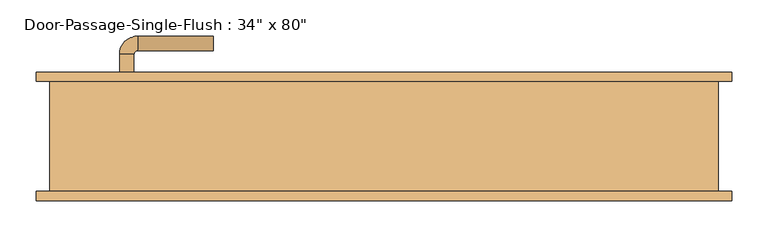
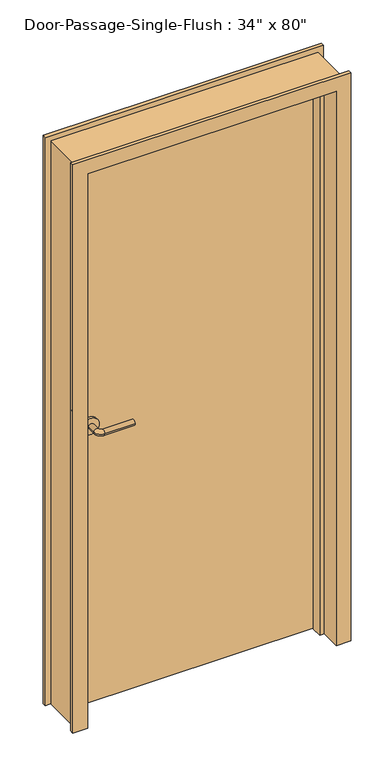
"""IFC4 building model written with IfcOpenShell, lengths in millimetres: door geometry."""

from ifc_helpers import new_model, si_unit, point, frame, frame_2d, origin, origin_with_axes, place, context, project, spatial, polyline, circle_curve, ellipse_curve, trimmed, segment, composite_curve, outline, extrude, faceted_brep, source, transform, mapped, element, save
from ifc_brep_helpers import plane_surface, cylinder_surface, revolved_surface, advanced_brep


def door_ade44093(model_context):
    return source(origin(), model_context, "Body", "SolidModel", [
        advanced_brep(
        [(-366.790625, 23.75, 1016.0), (-346.790625, 23.75, 1016.0), (-346.790625, -6.25, 1016.0), (-366.790625, -6.25, 1016.0), (-341.790625, -11.25, 1016.0), (-341.790625, -31.25, 1016.0), (-236.790625, -31.25, 1016.0), (-236.790625, -11.25, 1016.0)],
        [
            (0, 1, circle_curve(frame((-356.790625, 23.75, 1016.0), z_axis=(0.0, 1.0, 0.0), x_axis=(1.0, 0.0, 0.0)), 10.0)),
            (1, 0, circle_curve(frame((-356.790625, 23.75, 1016.0), z_axis=(0.0, 1.0, 0.0), x_axis=(1.0, 0.0, 0.0)), 10.0)),
            (1, 2),
            (2, 3, circle_curve(frame((-356.790625, -6.25, 1016.0), z_axis=(0.0, 1.0, 0.0), x_axis=(1.0, 0.0, 0.0)), 10.0)),
            (3, 0),
            (3, 2, circle_curve(frame((-356.790625, -6.25, 1016.0), z_axis=(0.0, 1.0, 0.0), x_axis=(1.0, 0.0, 0.0)), 10.0)),
            (4, 5, circle_curve(frame((-341.790625, -21.25, 1016.0), z_axis=(-1.0, 0.0, 0.0), x_axis=(0.0, 1.0, 0.0)), 10.0)),
            (5, 3, circle_curve(frame((-341.790625, -6.25, 1016.0), z_axis=(0.0, 0.0, -1.0), x_axis=(-1.0, 0.0, 0.0)), 25.0)),
            (2, 4, circle_curve(frame((-341.790625, -6.25, 1016.0), z_axis=(0.0, 0.0, 1.0), x_axis=(-1.0, 0.0, 0.0)), 5.0)),
            (5, 4, circle_curve(frame((-341.790625, -21.25, 1016.0), z_axis=(-1.0, 0.0, 0.0), x_axis=(0.0, 1.0, 0.0)), 10.0)),
            (6, 7, circle_curve(frame((-236.790625, -21.25, 1016.0), z_axis=(1.0, 0.0, 0.0), x_axis=(0.0, 1.0, 0.0)), 10.0)),
            (7, 6, circle_curve(frame((-236.790625, -21.25, 1016.0), z_axis=(1.0, 0.0, 0.0), x_axis=(0.0, 1.0, 0.0)), 10.0)),
            (4, 7),
            (6, 5),
        ],
        [
            plane_surface(frame((-356.790625, 23.75, 1016.0), z_axis=(0.0, 1.0, 0.0), x_axis=(0.0, 0.0, 1.0))),
            cylinder_surface(frame((-356.790625, 23.75, 1016.0), z_axis=(0.0, 1.0, 0.0), x_axis=(1.0, 0.0, 0.0)), 10.0),
            revolved_surface(trimmed(ellipse_curve(frame((-356.790625, -6.25, 1016.0), z_axis=(0.0, -1.0, 0.0), x_axis=(1.0, 0.0, 0.0)), 10.0, 10.0), [point((-366.790625, -6.25, 1016.0))], [point((-346.790625, -6.25, 1016.0))], True, "CARTESIAN"), (-341.790625, -6.25, 1016.0), (0.0, 0.0, -1.0)),
            revolved_surface(trimmed(ellipse_curve(frame((-356.790625, -6.25, 1016.0), z_axis=(0.0, -1.0, 0.0), x_axis=(1.0, 0.0, 0.0)), 10.0, 10.0), [point((-346.790625, -6.25, 1016.0))], [point((-366.790625, -6.25, 1016.0))], True, "CARTESIAN"), (-341.790625, -6.25, 1016.0), (0.0, 0.0, -1.0)),
            plane_surface(frame((-236.790625, -21.25, 1016.0), z_axis=(1.0, 0.0, 0.0), x_axis=(0.0, 0.0, 1.0))),
            cylinder_surface(frame((-341.790625, -21.25, 1016.0), z_axis=(-1.0, 0.0, 0.0), x_axis=(0.0, 1.0, 0.0)), 10.0),
        ],
        [
            (0, [[1, 2]]),
            (1, [[3, 4, 5, -2]]),
            (1, [[-5, 6, -3, -1]]),
            (2, [[7, 8, -4, 9]]),
            (3, [[10, -9, -6, -8]]),
            (4, [[11, 12]]),
            (5, [[13, -11, 14, -7]]),
            (5, [[-14, -12, -13, -10]]),
        ],
    ),
        extrude(outline(composite_curve([segment(trimmed(circle_curve(frame_2d((1016.0, -359.290625)), 30.0), [point((1016.0, -389.290625))], [point((1016.0, -329.290625))], False, "CARTESIAN"), True, "CONTINUOUS"), segment(trimmed(circle_curve(frame_2d((1016.0, -359.290625)), 30.0), [point((1016.0, -329.290625))], [point((1016.0, -389.290625))], False, "CARTESIAN"), True, "CONTINUOUS")], self_intersect=False)), frame((0.0, 23.75, 0.0), z_axis=(0.0, 1.0, 0.0), x_axis=(0.0, 0.0, 1.0)), (0.0, 0.0, 1.0), 8.0),
        advanced_brep(
        [(-366.790625, 90.55, 1016.0), (-346.790625, 90.55, 1016.0), (-366.790625, 120.55, 1016.0), (-346.790625, 120.55, 1016.0), (-341.790625, 125.55, 1016.0), (-341.790625, 145.55, 1016.0), (-236.790625, 145.55, 1016.0), (-236.790625, 125.55, 1016.0)],
        [
            (0, 1, circle_curve(frame((-356.790625, 90.55, 1016.0), z_axis=(0.0, -1.0, 0.0), x_axis=(1.0, 0.0, 0.0)), 10.0)),
            (1, 0, circle_curve(frame((-356.790625, 90.55, 1016.0), z_axis=(0.0, -1.0, 0.0), x_axis=(1.0, 0.0, 0.0)), 10.0)),
            (0, 2),
            (2, 3, circle_curve(frame((-356.790625, 120.55, 1016.0), z_axis=(0.0, -1.0, 0.0), x_axis=(1.0, 0.0, 0.0)), 10.0)),
            (3, 1),
            (3, 2, circle_curve(frame((-356.790625, 120.55, 1016.0), z_axis=(0.0, -1.0, 0.0), x_axis=(1.0, 0.0, 0.0)), 10.0)),
            (4, 3, circle_curve(frame((-341.790625, 120.55, 1016.0), z_axis=(0.0, 0.0, 1.0), x_axis=(-1.0, 0.0, 0.0)), 5.0)),
            (2, 5, circle_curve(frame((-341.790625, 120.55, 1016.0), z_axis=(0.0, 0.0, -1.0), x_axis=(-1.0, 0.0, 0.0)), 25.0)),
            (5, 4, circle_curve(frame((-341.790625, 135.55, 1016.0), z_axis=(-1.0, 0.0, 0.0), x_axis=(0.0, -1.0, 0.0)), 10.0)),
            (4, 5, circle_curve(frame((-341.790625, 135.55, 1016.0), z_axis=(-1.0, 0.0, 0.0), x_axis=(0.0, -1.0, 0.0)), 10.0)),
            (6, 7, circle_curve(frame((-236.790625, 135.55, 1016.0), z_axis=(1.0, 0.0, 0.0), x_axis=(0.0, -1.0, 0.0)), 10.0)),
            (7, 6, circle_curve(frame((-236.790625, 135.55, 1016.0), z_axis=(1.0, 0.0, 0.0), x_axis=(0.0, -1.0, 0.0)), 10.0)),
            (5, 6),
            (7, 4),
        ],
        [
            plane_surface(frame((-356.790625, 90.55, 1016.0), z_axis=(0.0, -1.0, 0.0), x_axis=(0.0, 0.0, 1.0))),
            cylinder_surface(frame((-356.790625, 90.55, 1016.0), z_axis=(0.0, -1.0, 0.0), x_axis=(1.0, 0.0, 0.0)), 10.0),
            revolved_surface(trimmed(ellipse_curve(frame((-356.790625, 120.55, 1016.0), z_axis=(0.0, -1.0, 0.0), x_axis=(1.0, 0.0, 0.0)), 10.0, 10.0), [point((-366.790625, 120.55, 1016.0))], [point((-346.790625, 120.55, 1016.0))], True, "CARTESIAN"), (-341.790625, 120.55, 1016.0), (0.0, 0.0, -1.0)),
            revolved_surface(trimmed(ellipse_curve(frame((-356.790625, 120.55, 1016.0), z_axis=(0.0, -1.0, 0.0), x_axis=(1.0, 0.0, 0.0)), 10.0, 10.0), [point((-346.790625, 120.55, 1016.0))], [point((-366.790625, 120.55, 1016.0))], True, "CARTESIAN"), (-341.790625, 120.55, 1016.0), (0.0, 0.0, -1.0)),
            plane_surface(frame((-236.790625, 135.55, 1016.0), z_axis=(1.0, 0.0, 0.0), x_axis=(0.0, 0.0, 1.0))),
            cylinder_surface(frame((-341.790625, 135.55, 1016.0), z_axis=(-1.0, 0.0, 0.0), x_axis=(0.0, -1.0, 0.0)), 10.0),
        ],
        [
            (0, [[1, 2]]),
            (1, [[-1, 3, 4, 5]]),
            (1, [[-2, -5, 6, -3]]),
            (2, [[7, -4, 8, 9]]),
            (3, [[-8, -6, -7, 10]]),
            (4, [[11, 12]]),
            (5, [[-9, 13, -12, 14]]),
            (5, [[-10, -14, -11, -13]]),
        ],
    ),
        extrude(outline(composite_curve([segment(trimmed(circle_curve(frame_2d((1016.0, -359.290625)), 30.0), [point((1016.0, -389.290625))], [point((1016.0, -329.290625))], False, "CARTESIAN"), True, "CONTINUOUS"), segment(trimmed(circle_curve(frame_2d((1016.0, -359.290625)), 30.0), [point((1016.0, -329.290625))], [point((1016.0, -389.290625))], False, "CARTESIAN"), True, "CONTINUOUS")], self_intersect=False)), frame((0.0, 82.55, 0.0), z_axis=(0.0, 1.0, 0.0), x_axis=(0.0, 0.0, 1.0)), (0.0, 0.0, 1.0), 8.0),
        faceted_brep([(431.8, 95.25, 0.0), (482.6, 95.25, 0.0), (482.6, 82.55, 0.0), (463.55, 82.55, 0.0), (463.55, -69.85, 0.0), (482.6, -69.85, 0.0), (482.6, -82.55, 0.0), (431.8, -82.55, 0.0), (431.8, -11.1125, 0.0), (415.925, -11.1125, 0.0), (415.925, 26.9875, 0.0), (431.8, 26.9875, 0.0), (431.8, 95.25, 2032.0), (-431.8, 95.25, 2032.0), (-431.8, 95.25, 0.0), (-482.6, 95.25, 0.0), (-482.6, 95.25, 2082.8), (482.6, 95.25, 2082.8), (482.6, 82.55, 2082.8), (-482.6, 82.55, 2082.8), (-482.6, 82.55, 0.0), (-463.55, 82.55, 0.0), (-463.55, 82.55, 2063.75), (463.55, 82.55, 2063.75), (463.55, -69.85, 2063.75), (-463.55, -69.85, 2063.75), (-463.55, -69.85, 0.0), (-482.6, -69.85, 0.0), (-482.6, -69.85, 2082.8), (482.6, -69.85, 2082.8), (482.6, -82.55, 2082.8), (-482.6, -82.55, 2082.8), (-482.6, -82.55, 0.0), (-431.8, -82.55, 0.0), (-431.8, -82.55, 2032.0), (431.8, -82.55, 2032.0), (431.8, -11.1125, 2032.0), (-431.8, -11.1125, 2032.0), (-431.8, -11.1125, 0.0), (-415.925, -11.1125, 0.0), (-415.925, -11.1125, 2016.125), (415.925, -11.1125, 2016.125), (415.925, 26.9875, 2016.125), (-415.925, 26.9875, 2016.125), (-415.925, 26.9875, 0.0), (-431.8, 26.9875, 0.0), (-431.8, 26.9875, 2032.0), (431.8, 26.9875, 2032.0)], [[[0, 1, 2, 3, 4, 5, 6, 7, 8, 9, 10, 11]], [[1, 0, 12, 13, 14, 15, 16, 17]], [[2, 1, 17, 18]], [[3, 2, 18, 19, 20, 21, 22, 23]], [[4, 3, 23, 24]], [[5, 4, 24, 25, 26, 27, 28, 29]], [[6, 5, 29, 30]], [[7, 6, 30, 31, 32, 33, 34, 35]], [[8, 7, 35, 36]], [[9, 8, 36, 37, 38, 39, 40, 41]], [[10, 9, 41, 42]], [[11, 10, 42, 43, 44, 45, 46, 47]], [[0, 11, 47, 12]], [[18, 17, 16, 19]], [[24, 23, 22, 25]], [[30, 29, 28, 31]], [[36, 35, 34, 37]], [[42, 41, 40, 43]], [[12, 47, 46, 13]], [[14, 45, 44, 39, 38, 33, 32, 27, 26, 21, 20, 15]], [[19, 16, 15, 20]], [[25, 22, 21, 26]], [[31, 28, 27, 32]], [[37, 34, 33, 38]], [[43, 40, 39, 44]], [[13, 46, 45, 14]]]),
        extrude(outline(polyline([(431.8, 31.75), (-431.8, 31.75), (-431.8, 82.55), (431.8, 82.55), (431.8, 31.75)])), origin_with_axes(), (0.0, 0.0, 1.0), 2032.0),
    ])


if __name__ == "__main__":
    model = new_model("IFC4")
    model_context = context("Model", 3, world=origin())
    ifc_project = project(units=[si_unit("LENGTHUNIT", "METRE", prefix="MILLI")], contexts=[model_context])
    site = spatial("IfcSite", under=ifc_project)
    building = spatial("IfcBuilding", under=site)
    placement = place(None, origin())
    door_shape = door_ade44093(model_context)
    element("IfcDoor", 1, ObjectType="Door-Passage-Single-Flush : 34\" x 80\"", at=placement, inside=building, context=model_context, shape_type="MappedRepresentation", body=[
        mapped(door_shape, transform((0.0, 0.0, 0.0), x_axis=(1.0, 0.0, 0.0), y_axis=(0.0, 1.0, 0.0), z_axis=(0.0, 0.0, 1.0))),
    ])
    save(model, "model.ifc")

# Revit data of these elements
# Type "Door-Passage-Single-Flush : 34\" x 80\""
#   Type Mark = "14"
#   Assembly Code = "C1020"
#   Analytic Construction = "Wooden"
#   Thickness = 0' - 2"
#   Thermal Resistance (R) = 2.5876 (h·ft²·°F)/BTU
#   Swing Angle [instance default] = 90.00°
#   Strike Height = 3' - 4"
#   Rough Width [instance default] = 3' - 2"
#   Rough Height [instance default] = 7' - 0"
#   Masonry Inset [instance default] = 0' - 1"
#   Masonry Frame Depth = 0' - 5 3/4"
#   MF Opening Width [instance default] = 0' - 4"
#   MF Opening Height [instance default] = 0' - 4"
#   Inset Calculate [instance default] = 0' - 4"
#   Heat Transfer Coefficient (U) = 0.3865 BTU/(h·ft²·°F)
#   Height = 6' - 8"
#   Width = 2' - 10"
#   Masonry Frame [instance default] = yes
#   Dry Wall Frame [instance default] = no
#   Panel Material = Wood - Birch
#   Door Handle Material = Aluminum
#   Frame Material = Door - Frame
#   Visual Light Transmittance = 0
#   Solar Heat Gain Coefficient = 0
#   Function = (empty or 0)
#   Wall Closure = (empty or 0)
# Element 1 (IfcDoor, "Door-Passage-Single-Flush : 34\" x 80\"")
#   Rough Width = 3' - 0 1/2"
#   Rough Height = 6' - 9 1/4"
#   MF Opening Width = 0' - 2 1/2"
#   MF Opening Height = 0' - 1 1/4"
#   Inset Calculate = 0' - 3"
#   Masonry Frame = no
#   Dry Wall Frame = yes
#   Materials on its faces: "Door - Frame", "Aluminum", "Wood - Birch"
# Materials
#   "Wood - Birch": class "Unassigned", colour RGB 224 178 126, transparency 0
#   "Aluminum": class "Metal", colour RGB 244 244 244, transparency 0, Description = "Aluminum 6061", Cost = 0
#   "Door - Frame": class "Unassigned", colour RGB 118 70 51, transparency 0
